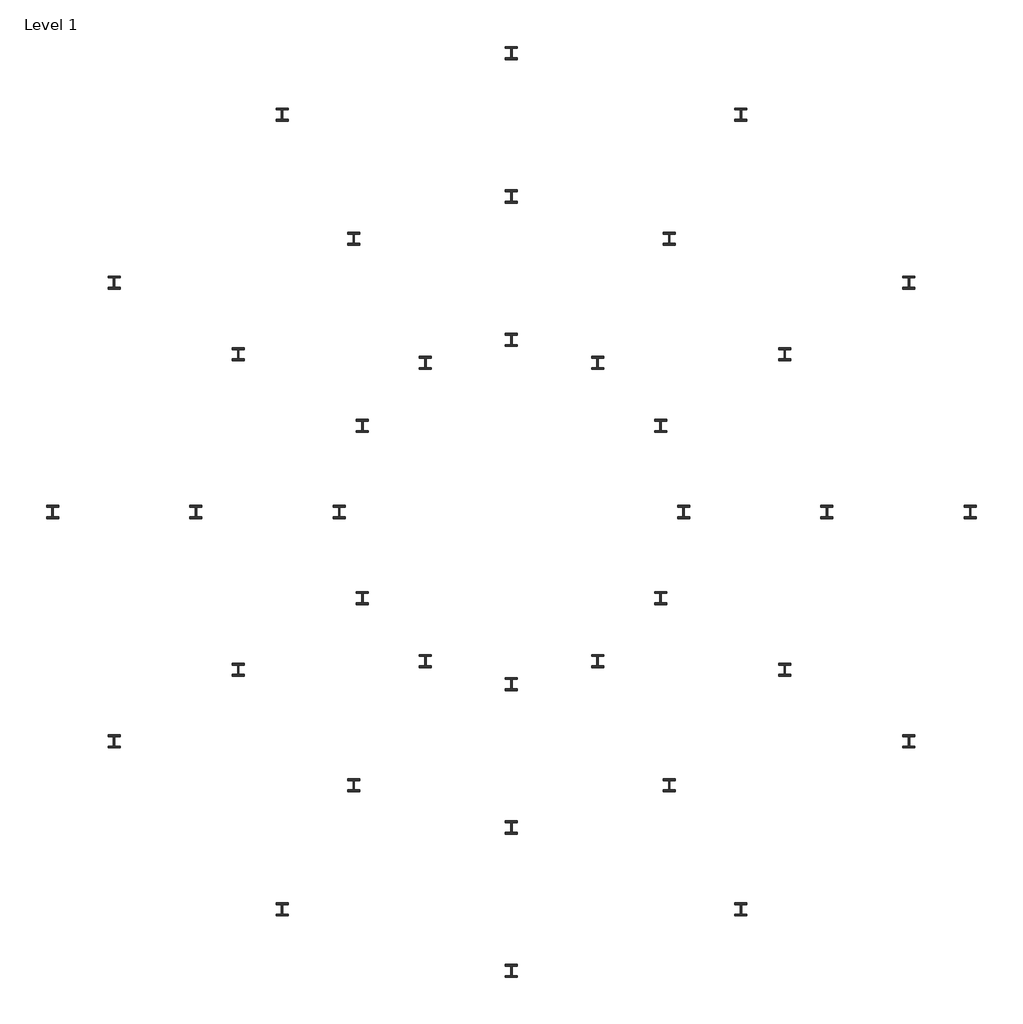
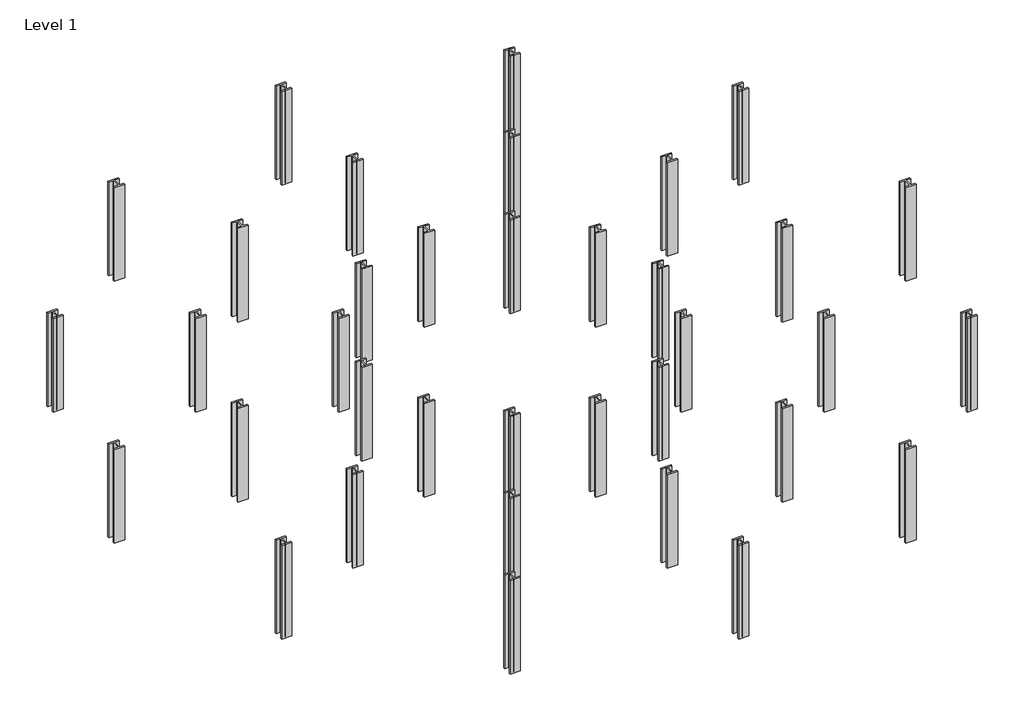
# One storey: 36 columns.
"""IFC4 building model written with IfcOpenShell, lengths in millimetres."""

import ifcopenshell
import ifcopenshell.guid

model = None  # the IFC model being written
_history = None  # IfcOwnerHistory: only IFC2X3 demands one
_inside = {}  # id of a spatial element -> (the spatial element, [elements in it])
_under = {}  # id of a project, library or spatial element -> (it, [spatial elements below it])
_declared = {}  # id of a project -> (the project, [libraries it declares])
_typed = {}  # id of a type object -> (the type object, [elements of that type])
_made_of = {}  # id of a material, layer set ... -> (it, [elements and type objects made of it])


def new_model(schema):
    """Start an empty IFC model of exactly this schema.

    Asked for "IFC4X3", IfcOpenShell would pick the latest addendum, in which some entities
    have other attributes; the version numbers below select the first issue.
    IFC2X3 requires an IfcOwnerHistory on every rooted entity: one is made here for all.
    """
    global model, _history
    if schema == "IFC4X3":
        model = ifcopenshell.file(schema_version=(4, 3, 0, 0))
    else:
        model = ifcopenshell.file(schema=schema)
    _inside.clear()
    _under.clear()
    _declared.clear()
    _typed.clear()
    _made_of.clear()
    _history = None
    if model.schema == "IFC2X3":
        org = make("IfcOrganization", Name="unknown")
        user = make(
            "IfcPersonAndOrganization",
            ThePerson=make("IfcPerson", FamilyName="unknown"),
            TheOrganization=org,
        )
        app = make(
            "IfcApplication",
            ApplicationDeveloper=org,
            Version="unknown",
            ApplicationFullName="unknown",
            ApplicationIdentifier="unknown",
        )
        _history = make(
            "IfcOwnerHistory",
            OwningUser=user,
            OwningApplication=app,
            ChangeAction="ADDED",
            CreationDate=0,
        )
    return model


def make(cls, **values):
    """One entity of the class cls with the attributes given. An attribute that is None is left unset."""
    return model.create_entity(
        cls, **{name: value for name, value in values.items() if value is not None}
    )


def rooted(cls, **values):
    """An entity with a GlobalId (a new one), such as an element, a storey or a relation."""
    return make(cls, GlobalId=ifcopenshell.guid.new(), OwnerHistory=_history, **values)


def si_unit(unit_type, name, prefix=None):
    """IfcSIUnit, for example si_unit("LENGTHUNIT", "METRE", prefix="MILLI")."""
    return make("IfcSIUnit", UnitType=unit_type, Prefix=prefix, Name=name)


def assignment(units):
    """IfcUnitAssignment: the units of a project."""
    return None if units is None else make("IfcUnitAssignment", Units=units)


def point(xyz):
    """IfcCartesianPoint."""
    return None if xyz is None else make("IfcCartesianPoint", Coordinates=xyz)


def direction(xyz):
    """IfcDirection."""
    return None if xyz is None else make("IfcDirection", DirectionRatios=xyz)


def frame(location, z_axis=None, x_axis=None):
    """IfcAxis2Placement3D, a coordinate frame: its origin and axes. An axis left out is left unset."""
    return make(
        "IfcAxis2Placement3D",
        Location=point(location),
        Axis=direction(z_axis),
        RefDirection=direction(x_axis),
    )


def frame_2d(location, x_axis=None):
    """IfcAxis2Placement2D, a coordinate frame in the plane: its origin and x axis."""
    return make(
        "IfcAxis2Placement2D", Location=point(location), RefDirection=direction(x_axis)
    )


def origin():
    """The frame at (0, 0, 0) with its axes left unset."""
    return frame((0.0, 0.0, 0.0))


def origin_with_axes():
    """The frame at (0, 0, 0) with the z axis (0, 0, 1) and the x axis (1, 0, 0) written out."""
    return frame((0.0, 0.0, 0.0), z_axis=(0.0, 0.0, 1.0), x_axis=(1.0, 0.0, 0.0))


def place(relative_to, where):
    """IfcLocalPlacement: puts the frame where relative to a parent placement (None: the world)."""
    return make(
        "IfcLocalPlacement", PlacementRelTo=relative_to, RelativePlacement=where
    )


def context(
    kind, dimensions, precision=None, world=None, true_north=None, identifier=None
):
    """IfcGeometricRepresentationContext, for example the 3D "Model" context."""
    return make(
        "IfcGeometricRepresentationContext",
        ContextIdentifier=identifier,
        ContextType=kind,
        CoordinateSpaceDimension=dimensions,
        Precision=precision,
        WorldCoordinateSystem=world,
        TrueNorth=true_north,
    )


def project(units=None, contexts=None):
    """IfcProject with its units and contexts."""
    return rooted(
        "IfcProject",
        Name="project",
        RepresentationContexts=contexts,
        UnitsInContext=assignment(units),
    )


def spatial(cls, under=None, at=None, **own):
    """A site, building, storey or space (cls), placed at a placement, below another one or the project."""
    s = rooted(cls, ObjectPlacement=at, **own)
    if under is not None:
        _under.setdefault(under.id(), (under, []))[1].append(s)
    return s


def polyline(points):
    """IfcPolyline through the points."""
    return make("IfcPolyline", Points=[point(p) for p in points])


def circle_curve(where, radius):
    """IfcCircle in the frame where."""
    return make("IfcCircle", Position=where, Radius=radius)


def trimmed(basis, trim1, trim2, sense, master):
    """IfcTrimmedCurve: the piece of a basis curve between two trims."""
    return make(
        "IfcTrimmedCurve",
        BasisCurve=basis,
        Trim1=trim1,
        Trim2=trim2,
        SenseAgreement=sense,
        MasterRepresentation=master,
    )


def segment(curve, same_sense, transition):
    """IfcCompositeCurveSegment."""
    return make(
        "IfcCompositeCurveSegment",
        Transition=transition,
        SameSense=same_sense,
        ParentCurve=curve,
    )


def composite_curve(segments, self_intersect=None):
    """IfcCompositeCurve: segments joined end to end."""
    return make("IfcCompositeCurve", Segments=segments, SelfIntersect=self_intersect)


def outline(outer, holes=None, kind="AREA"):
    """IfcArbitraryClosedProfileDef: a profile drawn as a closed curve; with holes, ...WithVoids."""
    if holes is None:
        return make("IfcArbitraryClosedProfileDef", ProfileType=kind, OuterCurve=outer)
    return make(
        "IfcArbitraryProfileDefWithVoids",
        ProfileType=kind,
        OuterCurve=outer,
        InnerCurves=holes,
    )


def extrude(swept, where, along, depth):
    """IfcExtrudedAreaSolid: the profile swept, set in the frame where, extruded along a direction by depth."""
    return make(
        "IfcExtrudedAreaSolid",
        SweptArea=swept,
        Position=where,
        ExtrudedDirection=direction(along),
        Depth=depth,
    )


def shape(context_of_items, identifier, shape_type, items):
    """IfcShapeRepresentation: the items that make up one representation, for example the "Body"."""
    return make(
        "IfcShapeRepresentation",
        ContextOfItems=context_of_items,
        RepresentationIdentifier=identifier,
        RepresentationType=shape_type,
        Items=items,
    )


def source(mapping_origin, context_of_items, identifier, shape_type, items):
    """IfcRepresentationMap: a shape defined once, which mapped items show again and again."""
    return make(
        "IfcRepresentationMap",
        MappingOrigin=mapping_origin,
        MappedRepresentation=shape(context_of_items, identifier, shape_type, items),
    )


def transform(
    local_origin,
    x_axis=None,
    y_axis=None,
    z_axis=None,
    scale=None,
    scale2=None,
    scale3=None,
    uniform=True,
):
    """IfcCartesianTransformationOperator3D, or its non-uniform kind. x_axis, y_axis, z_axis: its Axis1, 2, 3."""
    if uniform:
        return make(
            "IfcCartesianTransformationOperator3D",
            Axis1=direction(x_axis),
            Axis2=direction(y_axis),
            LocalOrigin=point(local_origin),
            Scale=scale,
            Axis3=direction(z_axis),
        )
    return make(
        "IfcCartesianTransformationOperator3DnonUniform",
        Axis1=direction(x_axis),
        Axis2=direction(y_axis),
        LocalOrigin=point(local_origin),
        Scale=scale,
        Axis3=direction(z_axis),
        Scale2=scale2,
        Scale3=scale3,
    )


def mapped(mapping_source, mapping_target):
    """IfcMappedItem: shows the shape of a source again, moved by a transform."""
    return make(
        "IfcMappedItem", MappingSource=mapping_source, MappingTarget=mapping_target
    )


def made_of(thing, what):
    """Note that an element or type object is made of a material, layer set ...; save() writes the relation."""
    if what is not None:
        _made_of.setdefault(what.id(), (what, []))[1].append(thing)
    return thing


def element(
    cls,
    number,
    at=None,
    inside=None,
    cuts=None,
    type_object=None,
    material=None,
    context=None,
    identifier="Body",
    shape_type=None,
    held_by="IfcProductDefinitionShape",
    body=None,
    shapes=None,
    **own,
):
    """One element of the class cls, such as IfcWall. Its Tag is "e" and its number.

    at: its placement. inside: the storey or other place that contains it. cuts: it is an
    opening in that element (IfcRelVoidsElement). A single representation is given by context,
    identifier, shape_type and body (its items); several are given by shapes. held_by: the class
    of the entity that holds the representations. save() writes the other relations.
    """
    e = rooted(cls, Tag="e%d" % number, ObjectPlacement=at, **own)
    if body is not None:
        shapes = [shape(context, identifier, shape_type, body)]
    if shapes is not None:
        e.Representation = make(held_by, Representations=shapes)
    if inside is not None:
        _inside.setdefault(inside.id(), (inside, []))[1].append(e)
    if cuts is not None:
        rooted(
            "IfcRelVoidsElement", RelatingBuildingElement=cuts, RelatedOpeningElement=e
        )
    if type_object is not None:
        _typed.setdefault(type_object.id(), (type_object, []))[1].append(e)
    return made_of(e, material)


def aggregate(whole, parts):
    """IfcRelAggregates: a whole, such as a stair, and the parts it consists of."""
    return rooted("IfcRelAggregates", RelatingObject=whole, RelatedObjects=parts)


def save(model, path):
    """Write the relations noted so far, then the file.

    IfcRelAggregates (storeys below a building ...), IfcRelContainedInSpatialStructure (elements
    in a storey), IfcRelDefinesByType, IfcRelAssociatesMaterial and IfcRelDeclares: one each for
    every whole, place, type object, material and project.
    """
    for whole, parts in _under.values():
        aggregate(whole, parts)
    for where, things in _inside.values():
        rooted(
            "IfcRelContainedInSpatialStructure",
            RelatedElements=things,
            RelatingStructure=where,
        )
    for kind, things in _typed.values():
        rooted("IfcRelDefinesByType", RelatedObjects=things, RelatingType=kind)
    for what, things in _made_of.values():
        rooted("IfcRelAssociatesMaterial", RelatedObjects=things, RelatingMaterial=what)
    for by, libraries in _declared.values():
        rooted("IfcRelDeclares", RelatingContext=by, RelatedDefinitions=libraries)
    model.write(path)


def uc_universal_columns_column_uc356x406x551_b8cfbe81(model_context):
    return source(origin(), model_context, "Body", "SweptSolid", [
        extrude(outline(composite_curve([segment(polyline([(209.25, 227.8), (209.25, 160.3), (36.25, 160.3)]), True, "CONTINUOUS"), segment(trimmed(circle_curve(frame_2d((36.25, 145.1)), 15.2), [point((36.25, 160.3))], [point((21.05, 145.1))], True, "CARTESIAN"), True, "CONTINUOUS"), segment(polyline([(21.05, 145.1), (21.05, -145.1)]), True, "CONTINUOUS"), segment(trimmed(circle_curve(frame_2d((36.25, -145.1)), 15.2), [point((21.05, -145.1))], [point((36.25, -160.3))], True, "CARTESIAN"), True, "CONTINUOUS"), segment(polyline([(36.25, -160.3), (209.25, -160.3), (209.25, -227.8), (-209.25, -227.8), (-209.25, -160.3), (-36.25, -160.3)]), True, "CONTINUOUS"), segment(trimmed(circle_curve(frame_2d((-36.25, -145.1)), 15.2), [point((-36.25, -160.3))], [point((-21.05, -145.1))], True, "CARTESIAN"), True, "CONTINUOUS"), segment(polyline([(-21.05, -145.1), (-21.05, 145.1)]), True, "CONTINUOUS"), segment(trimmed(circle_curve(frame_2d((-36.25, 145.1)), 15.2), [point((-21.05, 145.1))], [point((-36.25, 160.3))], True, "CARTESIAN"), True, "CONTINUOUS"), segment(polyline([(-36.25, 160.3), (-209.25, 160.3), (-209.25, 227.8), (209.25, 227.8)]), True, "CONTINUOUS")], self_intersect=False)), origin_with_axes(), (0.0, 0.0, 1.0), 4000.0),
    ])


model = new_model("IFC4")

# Units and contexts
model_context = context("Model", 3, world=origin())
ifc_project = project(units=[si_unit("LENGTHUNIT", "METRE", prefix="MILLI")], contexts=[model_context])

# Site, building, storey
site = spatial("IfcSite", under=ifc_project)
building = spatial("IfcBuilding", under=site)
storey = spatial("IfcBuildingStorey", under=building, Name="Level 1", Elevation=0.0)

# Columns
placement = place(None, origin())
uc_universal_columns_column_uc356x406x551_shape = uc_universal_columns_column_uc356x406x551_b8cfbe81(model_context)
element("IfcColumn", 1, ObjectType="UC-Universal Columns-Column : UC356x406x551", at=placement, inside=storey, context=model_context, shape_type="MappedRepresentation", body=[
    mapped(uc_universal_columns_column_uc356x406x551_shape, transform((6000.0, 0.0, 0.0), x_axis=(1.0, 0.0, 0.0), y_axis=(0.0, 1.0, 0.0), z_axis=(0.0, 0.0, 1.0))),
])
element("IfcColumn", 2, ObjectType="UC-Universal Columns-Column : UC356x406x551", at=placement, inside=storey, context=model_context, shape_type="MappedRepresentation", body=[
    mapped(uc_universal_columns_column_uc356x406x551_shape, transform((5196.1524227, 3000.0, 0.0), x_axis=(1.0, 0.0, 0.0), y_axis=(0.0, 1.0, 0.0), z_axis=(0.0, 0.0, 1.0))),
])
element("IfcColumn", 3, ObjectType="UC-Universal Columns-Column : UC356x406x551", at=placement, inside=storey, context=model_context, shape_type="MappedRepresentation", body=[
    mapped(uc_universal_columns_column_uc356x406x551_shape, transform((3000.0, 5196.1524227, 0.0), x_axis=(1.0, 0.0, 0.0), y_axis=(0.0, 1.0, 0.0), z_axis=(0.0, 0.0, 1.0))),
])
element("IfcColumn", 4, ObjectType="UC-Universal Columns-Column : UC356x406x551", at=placement, inside=storey, context=model_context, shape_type="MappedRepresentation", body=[
    mapped(uc_universal_columns_column_uc356x406x551_shape, transform((0.0, 6000.0, 0.0), x_axis=(1.0, 0.0, 0.0), y_axis=(0.0, 1.0, 0.0), z_axis=(0.0, 0.0, 1.0))),
])
element("IfcColumn", 5, ObjectType="UC-Universal Columns-Column : UC356x406x551", at=placement, inside=storey, context=model_context, shape_type="MappedRepresentation", body=[
    mapped(uc_universal_columns_column_uc356x406x551_shape, transform((-3000.0, 5196.1524227, 0.0), x_axis=(1.0, 0.0, 0.0), y_axis=(0.0, 1.0, 0.0), z_axis=(0.0, 0.0, 1.0))),
])
element("IfcColumn", 6, ObjectType="UC-Universal Columns-Column : UC356x406x551", at=placement, inside=storey, context=model_context, shape_type="MappedRepresentation", body=[
    mapped(uc_universal_columns_column_uc356x406x551_shape, transform((-5196.1524227, 3000.0, 0.0), x_axis=(1.0, 0.0, 0.0), y_axis=(0.0, 1.0, 0.0), z_axis=(0.0, 0.0, 1.0))),
])
element("IfcColumn", 7, ObjectType="UC-Universal Columns-Column : UC356x406x551", at=placement, inside=storey, context=model_context, shape_type="MappedRepresentation", body=[
    mapped(uc_universal_columns_column_uc356x406x551_shape, transform((-6000.0, 0.0, 0.0), x_axis=(1.0, 0.0, 0.0), y_axis=(0.0, 1.0, 0.0), z_axis=(0.0, 0.0, 1.0))),
])
element("IfcColumn", 8, ObjectType="UC-Universal Columns-Column : UC356x406x551", at=placement, inside=storey, context=model_context, shape_type="MappedRepresentation", body=[
    mapped(uc_universal_columns_column_uc356x406x551_shape, transform((-5196.1524227, -3000.0, 0.0), x_axis=(1.0, 0.0, 0.0), y_axis=(0.0, 1.0, 0.0), z_axis=(0.0, 0.0, 1.0))),
])
element("IfcColumn", 9, ObjectType="UC-Universal Columns-Column : UC356x406x551", at=placement, inside=storey, context=model_context, shape_type="MappedRepresentation", body=[
    mapped(uc_universal_columns_column_uc356x406x551_shape, transform((-3000.0, -5196.1524227, 0.0), x_axis=(1.0, 0.0, 0.0), y_axis=(0.0, 1.0, 0.0), z_axis=(0.0, 0.0, 1.0))),
])
element("IfcColumn", 10, ObjectType="UC-Universal Columns-Column : UC356x406x551", at=placement, inside=storey, context=model_context, shape_type="MappedRepresentation", body=[
    mapped(uc_universal_columns_column_uc356x406x551_shape, transform((0.0, -6000.0, 0.0), x_axis=(1.0, 0.0, 0.0), y_axis=(0.0, 1.0, 0.0), z_axis=(0.0, 0.0, 1.0))),
])
element("IfcColumn", 11, ObjectType="UC-Universal Columns-Column : UC356x406x551", at=placement, inside=storey, context=model_context, shape_type="MappedRepresentation", body=[
    mapped(uc_universal_columns_column_uc356x406x551_shape, transform((3000.0, -5196.1524227, 0.0), x_axis=(1.0, 0.0, 0.0), y_axis=(0.0, 1.0, 0.0), z_axis=(0.0, 0.0, 1.0))),
])
element("IfcColumn", 12, ObjectType="UC-Universal Columns-Column : UC356x406x551", at=placement, inside=storey, context=model_context, shape_type="MappedRepresentation", body=[
    mapped(uc_universal_columns_column_uc356x406x551_shape, transform((5196.1524227, -3000.0, 0.0), x_axis=(1.0, 0.0, 0.0), y_axis=(0.0, 1.0, 0.0), z_axis=(0.0, 0.0, 1.0))),
])
element("IfcColumn", 13, ObjectType="UC-Universal Columns-Column : UC356x406x551", at=placement, inside=storey, context=model_context, shape_type="MappedRepresentation", body=[
    mapped(uc_universal_columns_column_uc356x406x551_shape, transform((11000.0, 0.0, 0.0), x_axis=(1.0, 0.0, 0.0), y_axis=(0.0, 1.0, 0.0), z_axis=(0.0, 0.0, 1.0))),
])
element("IfcColumn", 14, ObjectType="UC-Universal Columns-Column : UC356x406x551", at=placement, inside=storey, context=model_context, shape_type="MappedRepresentation", body=[
    mapped(uc_universal_columns_column_uc356x406x551_shape, transform((9526.2794416, 5500.0, 0.0), x_axis=(1.0, 0.0, 0.0), y_axis=(0.0, 1.0, 0.0), z_axis=(0.0, 0.0, 1.0))),
])
element("IfcColumn", 15, ObjectType="UC-Universal Columns-Column : UC356x406x551", at=placement, inside=storey, context=model_context, shape_type="MappedRepresentation", body=[
    mapped(uc_universal_columns_column_uc356x406x551_shape, transform((5500.0, 9526.2794416, 0.0), x_axis=(1.0, 0.0, 0.0), y_axis=(0.0, 1.0, 0.0), z_axis=(0.0, 0.0, 1.0))),
])
element("IfcColumn", 16, ObjectType="UC-Universal Columns-Column : UC356x406x551", at=placement, inside=storey, context=model_context, shape_type="MappedRepresentation", body=[
    mapped(uc_universal_columns_column_uc356x406x551_shape, transform((0.0, 11000.0, 0.0), x_axis=(1.0, 0.0, 0.0), y_axis=(0.0, 1.0, 0.0), z_axis=(0.0, 0.0, 1.0))),
])
element("IfcColumn", 17, ObjectType="UC-Universal Columns-Column : UC356x406x551", at=placement, inside=storey, context=model_context, shape_type="MappedRepresentation", body=[
    mapped(uc_universal_columns_column_uc356x406x551_shape, transform((-5500.0, 9526.2794416, 0.0), x_axis=(1.0, 0.0, 0.0), y_axis=(0.0, 1.0, 0.0), z_axis=(0.0, 0.0, 1.0))),
])
element("IfcColumn", 18, ObjectType="UC-Universal Columns-Column : UC356x406x551", at=placement, inside=storey, context=model_context, shape_type="MappedRepresentation", body=[
    mapped(uc_universal_columns_column_uc356x406x551_shape, transform((-9526.2794416, 5500.0, 0.0), x_axis=(1.0, 0.0, 0.0), y_axis=(0.0, 1.0, 0.0), z_axis=(0.0, 0.0, 1.0))),
])
element("IfcColumn", 19, ObjectType="UC-Universal Columns-Column : UC356x406x551", at=placement, inside=storey, context=model_context, shape_type="MappedRepresentation", body=[
    mapped(uc_universal_columns_column_uc356x406x551_shape, transform((-11000.0, 0.0, 0.0), x_axis=(1.0, 0.0, 0.0), y_axis=(0.0, 1.0, 0.0), z_axis=(0.0, 0.0, 1.0))),
])
element("IfcColumn", 20, ObjectType="UC-Universal Columns-Column : UC356x406x551", at=placement, inside=storey, context=model_context, shape_type="MappedRepresentation", body=[
    mapped(uc_universal_columns_column_uc356x406x551_shape, transform((-9526.2794416, -5500.0, 0.0), x_axis=(1.0, 0.0, 0.0), y_axis=(0.0, 1.0, 0.0), z_axis=(0.0, 0.0, 1.0))),
])
element("IfcColumn", 21, ObjectType="UC-Universal Columns-Column : UC356x406x551", at=placement, inside=storey, context=model_context, shape_type="MappedRepresentation", body=[
    mapped(uc_universal_columns_column_uc356x406x551_shape, transform((-5500.0, -9526.2794416, 0.0), x_axis=(1.0, 0.0, 0.0), y_axis=(0.0, 1.0, 0.0), z_axis=(0.0, 0.0, 1.0))),
])
element("IfcColumn", 22, ObjectType="UC-Universal Columns-Column : UC356x406x551", at=placement, inside=storey, context=model_context, shape_type="MappedRepresentation", body=[
    mapped(uc_universal_columns_column_uc356x406x551_shape, transform((0.0, -11000.0, 0.0), x_axis=(1.0, 0.0, 0.0), y_axis=(0.0, 1.0, 0.0), z_axis=(0.0, 0.0, 1.0))),
])
element("IfcColumn", 23, ObjectType="UC-Universal Columns-Column : UC356x406x551", at=placement, inside=storey, context=model_context, shape_type="MappedRepresentation", body=[
    mapped(uc_universal_columns_column_uc356x406x551_shape, transform((5500.0, -9526.2794416, 0.0), x_axis=(1.0, 0.0, 0.0), y_axis=(0.0, 1.0, 0.0), z_axis=(0.0, 0.0, 1.0))),
])
element("IfcColumn", 24, ObjectType="UC-Universal Columns-Column : UC356x406x551", at=placement, inside=storey, context=model_context, shape_type="MappedRepresentation", body=[
    mapped(uc_universal_columns_column_uc356x406x551_shape, transform((9526.2794416, -5500.0, 0.0), x_axis=(1.0, 0.0, 0.0), y_axis=(0.0, 1.0, 0.0), z_axis=(0.0, 0.0, 1.0))),
])
element("IfcColumn", 25, ObjectType="UC-Universal Columns-Column : UC356x406x551", at=placement, inside=storey, context=model_context, shape_type="MappedRepresentation", body=[
    mapped(uc_universal_columns_column_uc356x406x551_shape, transform((16000.0, 0.0, 0.0), x_axis=(1.0, 0.0, 0.0), y_axis=(0.0, 1.0, 0.0), z_axis=(0.0, 0.0, 1.0))),
])
element("IfcColumn", 26, ObjectType="UC-Universal Columns-Column : UC356x406x551", at=placement, inside=storey, context=model_context, shape_type="MappedRepresentation", body=[
    mapped(uc_universal_columns_column_uc356x406x551_shape, transform((13856.4064606, 8000.0, 0.0), x_axis=(1.0, 0.0, 0.0), y_axis=(0.0, 1.0, 0.0), z_axis=(0.0, 0.0, 1.0))),
])
element("IfcColumn", 27, ObjectType="UC-Universal Columns-Column : UC356x406x551", at=placement, inside=storey, context=model_context, shape_type="MappedRepresentation", body=[
    mapped(uc_universal_columns_column_uc356x406x551_shape, transform((8000.0, 13856.4064606, 0.0), x_axis=(1.0, 0.0, 0.0), y_axis=(0.0, 1.0, 0.0), z_axis=(0.0, 0.0, 1.0))),
])
element("IfcColumn", 28, ObjectType="UC-Universal Columns-Column : UC356x406x551", at=placement, inside=storey, context=model_context, shape_type="MappedRepresentation", body=[
    mapped(uc_universal_columns_column_uc356x406x551_shape, transform((0.0, 16000.0, 0.0), x_axis=(1.0, 0.0, 0.0), y_axis=(0.0, 1.0, 0.0), z_axis=(0.0, 0.0, 1.0))),
])
element("IfcColumn", 29, ObjectType="UC-Universal Columns-Column : UC356x406x551", at=placement, inside=storey, context=model_context, shape_type="MappedRepresentation", body=[
    mapped(uc_universal_columns_column_uc356x406x551_shape, transform((-8000.0, 13856.4064606, 0.0), x_axis=(1.0, 0.0, 0.0), y_axis=(0.0, 1.0, 0.0), z_axis=(0.0, 0.0, 1.0))),
])
element("IfcColumn", 30, ObjectType="UC-Universal Columns-Column : UC356x406x551", at=placement, inside=storey, context=model_context, shape_type="MappedRepresentation", body=[
    mapped(uc_universal_columns_column_uc356x406x551_shape, transform((-13856.4064606, 8000.0, 0.0), x_axis=(1.0, 0.0, 0.0), y_axis=(0.0, 1.0, 0.0), z_axis=(0.0, 0.0, 1.0))),
])
element("IfcColumn", 31, ObjectType="UC-Universal Columns-Column : UC356x406x551", at=placement, inside=storey, context=model_context, shape_type="MappedRepresentation", body=[
    mapped(uc_universal_columns_column_uc356x406x551_shape, transform((-16000.0, 0.0, 0.0), x_axis=(1.0, 0.0, 0.0), y_axis=(0.0, 1.0, 0.0), z_axis=(0.0, 0.0, 1.0))),
])
element("IfcColumn", 32, ObjectType="UC-Universal Columns-Column : UC356x406x551", at=placement, inside=storey, context=model_context, shape_type="MappedRepresentation", body=[
    mapped(uc_universal_columns_column_uc356x406x551_shape, transform((-13856.4064606, -8000.0, 0.0), x_axis=(1.0, 0.0, 0.0), y_axis=(0.0, 1.0, 0.0), z_axis=(0.0, 0.0, 1.0))),
])
element("IfcColumn", 33, ObjectType="UC-Universal Columns-Column : UC356x406x551", at=placement, inside=storey, context=model_context, shape_type="MappedRepresentation", body=[
    mapped(uc_universal_columns_column_uc356x406x551_shape, transform((-8000.0, -13856.4064606, 0.0), x_axis=(1.0, 0.0, 0.0), y_axis=(0.0, 1.0, 0.0), z_axis=(0.0, 0.0, 1.0))),
])
element("IfcColumn", 34, ObjectType="UC-Universal Columns-Column : UC356x406x551", at=placement, inside=storey, context=model_context, shape_type="MappedRepresentation", body=[
    mapped(uc_universal_columns_column_uc356x406x551_shape, transform((0.0, -16000.0, 0.0), x_axis=(1.0, 0.0, 0.0), y_axis=(0.0, 1.0, 0.0), z_axis=(0.0, 0.0, 1.0))),
])
element("IfcColumn", 35, ObjectType="UC-Universal Columns-Column : UC356x406x551", at=placement, inside=storey, context=model_context, shape_type="MappedRepresentation", body=[
    mapped(uc_universal_columns_column_uc356x406x551_shape, transform((8000.0, -13856.4064606, 0.0), x_axis=(1.0, 0.0, 0.0), y_axis=(0.0, 1.0, 0.0), z_axis=(0.0, 0.0, 1.0))),
])
element("IfcColumn", 36, ObjectType="UC-Universal Columns-Column : UC356x406x551", at=placement, inside=storey, context=model_context, shape_type="MappedRepresentation", body=[
    mapped(uc_universal_columns_column_uc356x406x551_shape, transform((13856.4064606, -8000.0, 0.0), x_axis=(1.0, 0.0, 0.0), y_axis=(0.0, 1.0, 0.0), z_axis=(0.0, 0.0, 1.0))),
])

save(model, "model.ifc")

# Revit data of these elements
# Project information
#   Project Issue Date = "Issue Date"
#   Project Status = "Project Status"
#   Client Name = "Owner"
#   Project Address = "Enter address here"
#   Project Name = "Project Name"
#   Project Number = "Project Number"
# Type "UC-Universal Columns-Column : UC356x406x551"
#   Section Name Key = "UC356x406x551"
#   Width = 41.85 cm
#   Web Thickness = 4.21 cm
#   Web Fillet = 1.52 cm
#   Warping Constant = 31100000.0 cm⁶
#   Torsional Moment of Inertia = 9240.00 cm⁴
#   Section Area = 702.0 cm²
#   Plastic Modulus weak axis = 6058.0 cm³
#   Plastic Modulus strong axis = 12076.0 cm³
#   Nominal Weight = 551.00 kgf/m
#   Moment of Inertia weak axis = 82671.00 cm⁴
#   Moment of Inertia strong axis = 226938.00 cm⁴
#   Height = 45.56 cm
#   Flange Thickness = 6.75 cm
#   Elastic Modulus weak axis = 3951.0 cm³
#   Elastic Modulus strong axis = 9962.0 cm³
#   Centroid Vertical = 22.78 cm
#   Centroid Horizontal = 20.925 cm
#   built-in parameter 1005541 = 0.246063 (stored number, unit not read)
#   built-in parameter 1005540 = 0.459318 (stored number, unit not read)
#   Bolt Spacing = 14.0 cm
#   Structural Material [instance default] = Metal - Steel 43-275
#   Type Comments = ""
#   Assembly Code = ""
# Elements 1, 2, 3, 4, 5, 6, 7, 8, 9, 10, 11, 12, 13, 14, 15, 16, 17, 18, 19, 20, 21, 22, 23, 24, 25, 26, 27, 28, 29, 30, 31, 32, 33, 34, 35, 36 (IfcColumn, "UC-Universal Columns-Column : UC356x406x551")
#   Structural Material = Metal - Steel 43-275
#   Phase Created = New Construction
#   Materials on its faces: "Metal - Steel 43-275"
# Materials
#   "Metal - Steel 43-275": class "Metal", colour RGB 247 247 247, transparency 0, Cost = 0
